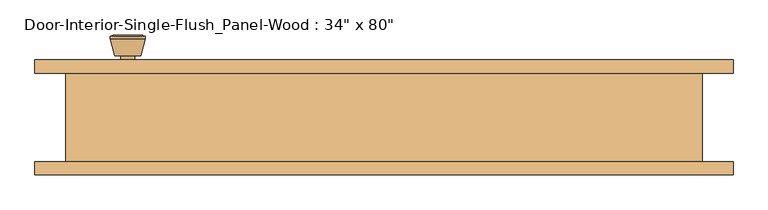
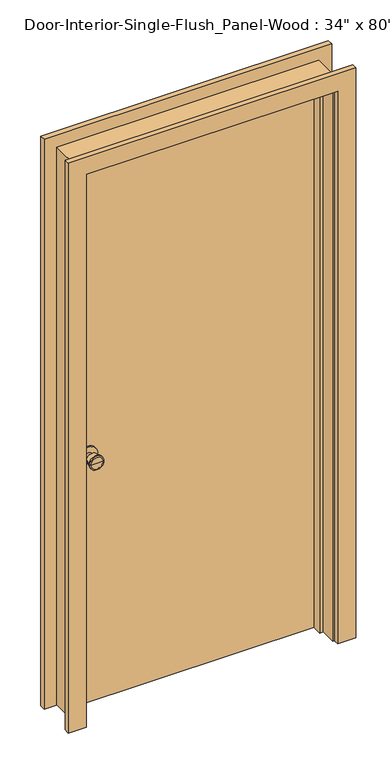
"""IFC4 building model written with IfcOpenShell, lengths in millimetres: door geometry."""

import ifcopenshell
import ifcopenshell.guid

model = None  # the IFC model being written
_history = None  # IfcOwnerHistory: only IFC2X3 demands one
_inside = {}  # id of a spatial element -> (the spatial element, [elements in it])
_under = {}  # id of a project, library or spatial element -> (it, [spatial elements below it])
_declared = {}  # id of a project -> (the project, [libraries it declares])
_typed = {}  # id of a type object -> (the type object, [elements of that type])
_made_of = {}  # id of a material, layer set ... -> (it, [elements and type objects made of it])


def new_model(schema):
    """Start an empty IFC model of exactly this schema.

    Asked for "IFC4X3", IfcOpenShell would pick the latest addendum, in which some entities
    have other attributes; the version numbers below select the first issue.
    IFC2X3 requires an IfcOwnerHistory on every rooted entity: one is made here for all.
    """
    global model, _history
    if schema == "IFC4X3":
        model = ifcopenshell.file(schema_version=(4, 3, 0, 0))
    else:
        model = ifcopenshell.file(schema=schema)
    _inside.clear()
    _under.clear()
    _declared.clear()
    _typed.clear()
    _made_of.clear()
    _history = None
    if model.schema == "IFC2X3":
        org = make("IfcOrganization", Name="unknown")
        user = make(
            "IfcPersonAndOrganization",
            ThePerson=make("IfcPerson", FamilyName="unknown"),
            TheOrganization=org,
        )
        app = make(
            "IfcApplication",
            ApplicationDeveloper=org,
            Version="unknown",
            ApplicationFullName="unknown",
            ApplicationIdentifier="unknown",
        )
        _history = make(
            "IfcOwnerHistory",
            OwningUser=user,
            OwningApplication=app,
            ChangeAction="ADDED",
            CreationDate=0,
        )
    return model


def make(cls, **values):
    """One entity of the class cls with the attributes given. An attribute that is None is left unset."""
    return model.create_entity(
        cls, **{name: value for name, value in values.items() if value is not None}
    )


def rooted(cls, **values):
    """An entity with a GlobalId (a new one), such as an element, a storey or a relation."""
    return make(cls, GlobalId=ifcopenshell.guid.new(), OwnerHistory=_history, **values)


def si_unit(unit_type, name, prefix=None):
    """IfcSIUnit, for example si_unit("LENGTHUNIT", "METRE", prefix="MILLI")."""
    return make("IfcSIUnit", UnitType=unit_type, Prefix=prefix, Name=name)


def assignment(units):
    """IfcUnitAssignment: the units of a project."""
    return None if units is None else make("IfcUnitAssignment", Units=units)


def point(xyz):
    """IfcCartesianPoint."""
    return None if xyz is None else make("IfcCartesianPoint", Coordinates=xyz)


def direction(xyz):
    """IfcDirection."""
    return None if xyz is None else make("IfcDirection", DirectionRatios=xyz)


def frame(location, z_axis=None, x_axis=None):
    """IfcAxis2Placement3D, a coordinate frame: its origin and axes. An axis left out is left unset."""
    return make(
        "IfcAxis2Placement3D",
        Location=point(location),
        Axis=direction(z_axis),
        RefDirection=direction(x_axis),
    )


def frame_2d(location, x_axis=None):
    """IfcAxis2Placement2D, a coordinate frame in the plane: its origin and x axis."""
    return make(
        "IfcAxis2Placement2D", Location=point(location), RefDirection=direction(x_axis)
    )


def origin():
    """The frame at (0, 0, 0) with its axes left unset."""
    return frame((0.0, 0.0, 0.0))


def origin_with_axes():
    """The frame at (0, 0, 0) with the z axis (0, 0, 1) and the x axis (1, 0, 0) written out."""
    return frame((0.0, 0.0, 0.0), z_axis=(0.0, 0.0, 1.0), x_axis=(1.0, 0.0, 0.0))


def place(relative_to, where):
    """IfcLocalPlacement: puts the frame where relative to a parent placement (None: the world)."""
    return make(
        "IfcLocalPlacement", PlacementRelTo=relative_to, RelativePlacement=where
    )


def context(
    kind, dimensions, precision=None, world=None, true_north=None, identifier=None
):
    """IfcGeometricRepresentationContext, for example the 3D "Model" context."""
    return make(
        "IfcGeometricRepresentationContext",
        ContextIdentifier=identifier,
        ContextType=kind,
        CoordinateSpaceDimension=dimensions,
        Precision=precision,
        WorldCoordinateSystem=world,
        TrueNorth=true_north,
    )


def project(units=None, contexts=None):
    """IfcProject with its units and contexts."""
    return rooted(
        "IfcProject",
        Name="project",
        RepresentationContexts=contexts,
        UnitsInContext=assignment(units),
    )


def spatial(cls, under=None, at=None, **own):
    """A site, building, storey or space (cls), placed at a placement, below another one or the project."""
    s = rooted(cls, ObjectPlacement=at, **own)
    if under is not None:
        _under.setdefault(under.id(), (under, []))[1].append(s)
    return s


def polyline(points):
    """IfcPolyline through the points."""
    return make("IfcPolyline", Points=[point(p) for p in points])


def circle_curve(where, radius):
    """IfcCircle in the frame where."""
    return make("IfcCircle", Position=where, Radius=radius)


def trimmed(basis, trim1, trim2, sense, master):
    """IfcTrimmedCurve: the piece of a basis curve between two trims."""
    return make(
        "IfcTrimmedCurve",
        BasisCurve=basis,
        Trim1=trim1,
        Trim2=trim2,
        SenseAgreement=sense,
        MasterRepresentation=master,
    )


def segment(curve, same_sense, transition):
    """IfcCompositeCurveSegment."""
    return make(
        "IfcCompositeCurveSegment",
        Transition=transition,
        SameSense=same_sense,
        ParentCurve=curve,
    )


def composite_curve(segments, self_intersect=None):
    """IfcCompositeCurve: segments joined end to end."""
    return make("IfcCompositeCurve", Segments=segments, SelfIntersect=self_intersect)


def outline(outer, holes=None, kind="AREA"):
    """IfcArbitraryClosedProfileDef: a profile drawn as a closed curve; with holes, ...WithVoids."""
    if holes is None:
        return make("IfcArbitraryClosedProfileDef", ProfileType=kind, OuterCurve=outer)
    return make(
        "IfcArbitraryProfileDefWithVoids",
        ProfileType=kind,
        OuterCurve=outer,
        InnerCurves=holes,
    )


def extrude(swept, where, along, depth):
    """IfcExtrudedAreaSolid: the profile swept, set in the frame where, extruded along a direction by depth."""
    return make(
        "IfcExtrudedAreaSolid",
        SweptArea=swept,
        Position=where,
        ExtrudedDirection=direction(along),
        Depth=depth,
    )


def faces_of(points, faces, orient=None, outer=None):
    """IfcFace entities. A face is a list of loops; a loop is a list of indices into points, from 0.

    orient and outer hold one flag for each loop. By default every Orientation is true, the
    first loop of a face is its IfcFaceOuterBound and the others are IfcFaceBound.
    """
    made = []
    for i, loops in enumerate(faces):
        bounds = []
        for j, loop in enumerate(loops):
            is_outer = j == 0 if outer is None else outer[i][j]
            bounds.append(
                make(
                    "IfcFaceOuterBound" if is_outer else "IfcFaceBound",
                    Bound=make("IfcPolyLoop", Polygon=[points[k] for k in loop]),
                    Orientation=True if orient is None else orient[i][j],
                )
            )
        made.append(make("IfcFace", Bounds=bounds))
    return made


def faceted_brep(points, faces, orient=None, outer=None, voids=None):
    """IfcFacetedBrep: a solid bounded by flat faces; with voids (closed shells), ...WithVoids."""
    shared = [point(p) for p in points]
    hull = make("IfcClosedShell", CfsFaces=faces_of(shared, faces, orient, outer))
    if voids is None:
        return make("IfcFacetedBrep", Outer=hull)
    return make(
        "IfcFacetedBrepWithVoids",
        Outer=hull,
        Voids=[
            make(cls, CfsFaces=faces_of(shared, fs, o, b)) for cls, fs, o, b in voids
        ],
    )


def shape(context_of_items, identifier, shape_type, items):
    """IfcShapeRepresentation: the items that make up one representation, for example the "Body"."""
    return make(
        "IfcShapeRepresentation",
        ContextOfItems=context_of_items,
        RepresentationIdentifier=identifier,
        RepresentationType=shape_type,
        Items=items,
    )


def source(mapping_origin, context_of_items, identifier, shape_type, items):
    """IfcRepresentationMap: a shape defined once, which mapped items show again and again."""
    return make(
        "IfcRepresentationMap",
        MappingOrigin=mapping_origin,
        MappedRepresentation=shape(context_of_items, identifier, shape_type, items),
    )


def transform(
    local_origin,
    x_axis=None,
    y_axis=None,
    z_axis=None,
    scale=None,
    scale2=None,
    scale3=None,
    uniform=True,
):
    """IfcCartesianTransformationOperator3D, or its non-uniform kind. x_axis, y_axis, z_axis: its Axis1, 2, 3."""
    if uniform:
        return make(
            "IfcCartesianTransformationOperator3D",
            Axis1=direction(x_axis),
            Axis2=direction(y_axis),
            LocalOrigin=point(local_origin),
            Scale=scale,
            Axis3=direction(z_axis),
        )
    return make(
        "IfcCartesianTransformationOperator3DnonUniform",
        Axis1=direction(x_axis),
        Axis2=direction(y_axis),
        LocalOrigin=point(local_origin),
        Scale=scale,
        Axis3=direction(z_axis),
        Scale2=scale2,
        Scale3=scale3,
    )


def mapped(mapping_source, mapping_target):
    """IfcMappedItem: shows the shape of a source again, moved by a transform."""
    return make(
        "IfcMappedItem", MappingSource=mapping_source, MappingTarget=mapping_target
    )


def made_of(thing, what):
    """Note that an element or type object is made of a material, layer set ...; save() writes the relation."""
    if what is not None:
        _made_of.setdefault(what.id(), (what, []))[1].append(thing)
    return thing


def element(
    cls,
    number,
    at=None,
    inside=None,
    cuts=None,
    type_object=None,
    material=None,
    context=None,
    identifier="Body",
    shape_type=None,
    held_by="IfcProductDefinitionShape",
    body=None,
    shapes=None,
    **own,
):
    """One element of the class cls, such as IfcWall. Its Tag is "e" and its number.

    at: its placement. inside: the storey or other place that contains it. cuts: it is an
    opening in that element (IfcRelVoidsElement). A single representation is given by context,
    identifier, shape_type and body (its items); several are given by shapes. held_by: the class
    of the entity that holds the representations. save() writes the other relations.
    """
    e = rooted(cls, Tag="e%d" % number, ObjectPlacement=at, **own)
    if body is not None:
        shapes = [shape(context, identifier, shape_type, body)]
    if shapes is not None:
        e.Representation = make(held_by, Representations=shapes)
    if inside is not None:
        _inside.setdefault(inside.id(), (inside, []))[1].append(e)
    if cuts is not None:
        rooted(
            "IfcRelVoidsElement", RelatingBuildingElement=cuts, RelatedOpeningElement=e
        )
    if type_object is not None:
        _typed.setdefault(type_object.id(), (type_object, []))[1].append(e)
    return made_of(e, material)


def aggregate(whole, parts):
    """IfcRelAggregates: a whole, such as a stair, and the parts it consists of."""
    return rooted("IfcRelAggregates", RelatingObject=whole, RelatedObjects=parts)


def save(model, path):
    """Write the relations noted so far, then the file.

    IfcRelAggregates (storeys below a building ...), IfcRelContainedInSpatialStructure (elements
    in a storey), IfcRelDefinesByType, IfcRelAssociatesMaterial and IfcRelDeclares: one each for
    every whole, place, type object, material and project.
    """
    for whole, parts in _under.values():
        aggregate(whole, parts)
    for where, things in _inside.values():
        rooted(
            "IfcRelContainedInSpatialStructure",
            RelatedElements=things,
            RelatingStructure=where,
        )
    for kind, things in _typed.values():
        rooted("IfcRelDefinesByType", RelatedObjects=things, RelatingType=kind)
    for what, things in _made_of.values():
        rooted("IfcRelAssociatesMaterial", RelatedObjects=things, RelatingMaterial=what)
    for by, libraries in _declared.values():
        rooted("IfcRelDeclares", RelatingContext=by, RelatedDefinitions=libraries)
    model.write(path)


def plane_surface(at):
    """IfcPlane: the flat surface through the origin of the frame at, square to its z axis."""
    return make("IfcPlane", Position=at)


def cylinder_surface(at, radius):
    """IfcCylindricalSurface: all points at the distance radius from the z axis of the frame at."""
    return make("IfcCylindricalSurface", Position=at, Radius=radius)


def revolved_surface(curve, axis_point, axis_direction):
    """IfcSurfaceOfRevolution: the curve turned about the line through axis_point along axis_direction."""
    return make(
        "IfcSurfaceOfRevolution",
        SweptCurve=make("IfcArbitraryOpenProfileDef", ProfileType="CURVE", Curve=curve),
        AxisPosition=make("IfcAxis1Placement", Location=point(axis_point), Axis=direction(axis_direction)),
    )


def advanced_brep(points, edges, surfaces, faces):
    """IfcAdvancedBrep: a solid bounded by faces that lie on surfaces and meet in shared edges.

    An edge is (start, end): straight between two places in points (the first is 0);
    or (start, end, curve); or (start, end, curve, False) where it runs against its curve.
    A face is (place in surfaces, loops), or (place, loops, False) where it looks against
    its surface's normal. A loop lists edges by number (the first is 1), with a minus sign
    where the edge is run from its end to its start. The first loop is the outer one.
    """
    corners = [point(p) for p in points]
    vertices = [make("IfcVertexPoint", VertexGeometry=c) for c in corners]
    made = []
    for start, end, *more in edges:
        made.append(
            make(
                "IfcEdgeCurve",
                EdgeStart=vertices[start],
                EdgeEnd=vertices[end],
                EdgeGeometry=more[0] if more else make("IfcPolyline", Points=[corners[start], corners[end]]),
                SameSense=more[1] if len(more) > 1 else True,
            )
        )
    hull = []
    for where, loops, *sense in faces:
        bounds = []
        for j, loop in enumerate(loops):
            ring = [make("IfcOrientedEdge", EdgeElement=made[abs(k) - 1], Orientation=k > 0) for k in loop]
            bounds.append(
                make(
                    "IfcFaceOuterBound" if j == 0 else "IfcFaceBound",
                    Bound=make("IfcEdgeLoop", EdgeList=ring),
                    Orientation=True,
                )
            )
        hull.append(make("IfcAdvancedFace", Bounds=bounds, FaceSurface=surfaces[where], SameSense=sense[0] if sense else True))
    return make("IfcAdvancedBrep", Outer=make("IfcClosedShell", CfsFaces=hull))


def door_5c12c2c5(model_context):
    return source(origin(), model_context, "Body", "SolidModel", [
        advanced_brep(
        [(-368.3, 19.4, 914.4), (-358.3, 19.4, 914.4), (-378.3, 19.4, 914.4), (-347.8241324, -29.6, 914.4), (-368.3, -29.6, 914.4), (-388.7758676, -29.6, 914.4), (-343.3, -27.7721319, 914.4), (-393.3, -27.7721319, 914.4), (-343.3, -24.3084537, 914.4), (-393.3, -24.3084537, 914.4), (-349.663764, 0.4, 914.4), (-386.936236, 0.4, 914.4), (-358.3, 0.4, 914.4), (-378.3, 0.4, 914.4)],
        [
            (0, 1),
            (1, 2, circle_curve(frame((-368.3, 19.4, 914.4), z_axis=(0.0, 1.0, 0.0), x_axis=(-1.0, 0.0, 0.0)), 10.0)),
            (2, 0),
            (2, 1, circle_curve(frame((-368.3, 19.4, 914.4), z_axis=(0.0, 1.0, 0.0), x_axis=(-1.0, 0.0, 0.0)), 10.0)),
            (3, 4),
            (4, 5),
            (5, 3, circle_curve(frame((-368.3, -29.6, 914.4), z_axis=(0.0, -1.0, 0.0), x_axis=(-1.0, 0.0, 0.0)), 20.4758676)),
            (3, 5, circle_curve(frame((-368.3, -29.6, 914.4), z_axis=(0.0, -1.0, 0.0), x_axis=(-1.0, 0.0, 0.0)), 20.4758676)),
            (6, 3),
            (5, 7),
            (7, 6, circle_curve(frame((-368.3, -27.7721319, 914.4), z_axis=(0.0, -1.0, 0.0), x_axis=(-1.0, 0.0, 0.0)), 25.0)),
            (6, 7, circle_curve(frame((-368.3, -27.7721319, 914.4), z_axis=(0.0, -1.0, 0.0), x_axis=(-1.0, 0.0, 0.0)), 25.0)),
            (8, 6),
            (7, 9),
            (9, 8, circle_curve(frame((-368.3, -24.3084537, 914.4), z_axis=(0.0, -1.0, 0.0), x_axis=(-1.0, 0.0, 0.0)), 25.0)),
            (8, 9, circle_curve(frame((-368.3, -24.3084537, 914.4), z_axis=(0.0, -1.0, 0.0), x_axis=(-1.0, 0.0, 0.0)), 25.0)),
            (10, 8),
            (9, 11),
            (11, 10, circle_curve(frame((-368.3, 0.4, 914.4), z_axis=(0.0, -1.0, 0.0), x_axis=(-1.0, 0.0, 0.0)), 18.636236)),
            (10, 11, circle_curve(frame((-368.3, 0.4, 914.4), z_axis=(0.0, -1.0, 0.0), x_axis=(-1.0, 0.0, 0.0)), 18.636236)),
            (12, 10),
            (11, 13),
            (13, 12, circle_curve(frame((-368.3, 0.4, 914.4), z_axis=(0.0, -1.0, 0.0), x_axis=(-1.0, 0.0, 0.0)), 10.0)),
            (12, 13, circle_curve(frame((-368.3, 0.4, 914.4), z_axis=(0.0, -1.0, 0.0), x_axis=(-1.0, 0.0, 0.0)), 10.0)),
            (1, 12),
            (13, 2),
        ],
        [
            plane_surface(frame((-368.3, 19.4, 914.4), z_axis=(0.0, 1.0, 0.0), x_axis=(-1.0, 0.0, 0.0))),
            plane_surface(frame((-368.3, -29.6, 914.4), z_axis=(0.0, -1.0, 0.0), x_axis=(-1.0, 0.0, 0.0))),
            revolved_surface(polyline([(-388.7758676, -29.6, 914.4), (-393.3, -27.7721319, 914.4)]), (-368.3, 19.4, 914.4), (0.0, 1.0, 0.0)),
            cylinder_surface(frame((-368.3, 19.4, 914.4), z_axis=(0.0, 1.0, 0.0), x_axis=(-1.0, 0.0, 0.0)), 25.0),
            revolved_surface(polyline([(-393.3, -24.3084537, 914.4), (-386.936236, 0.4, 914.4)]), (-368.3, 19.4, 914.4), (0.0, 1.0, 0.0)),
            plane_surface(frame((-368.3, 0.4, 914.4), z_axis=(0.0, 1.0, 0.0), x_axis=(-1.0, 0.0, 0.0))),
            cylinder_surface(frame((-368.3, 19.4, 914.4), z_axis=(0.0, 1.0, 0.0), x_axis=(-1.0, 0.0, 0.0)), 10.0),
        ],
        [
            (0, [[1, 2, 3]]),
            (0, [[-3, 4, -1]]),
            (1, [[5, 6, 7]]),
            (1, [[-6, -5, 8]]),
            (2, [[9, -7, 10, 11]]),
            (2, [[-10, -8, -9, 12]]),
            (3, [[13, -11, 14, 15]]),
            (3, [[-14, -12, -13, 16]]),
            (4, [[17, -15, 18, 19]]),
            (4, [[-18, -16, -17, 20]]),
            (5, [[21, -19, 22, 23]]),
            (5, [[-22, -20, -21, 24]]),
            (6, [[25, -23, 26, -2]]),
            (6, [[-26, -24, -25, -4]]),
        ],
    ),
        extrude(outline(composite_curve([segment(trimmed(circle_curve(frame_2d((914.4, -368.3)), 30.0), [point((914.4, -398.3))], [point((914.4, -338.3))], False, "CARTESIAN"), True, "CONTINUOUS"), segment(trimmed(circle_curve(frame_2d((914.4, -368.3)), 30.0), [point((914.4, -338.3))], [point((914.4, -398.3))], False, "CARTESIAN"), True, "CONTINUOUS")], self_intersect=False)), frame((0.0, 19.4, 0.0), z_axis=(0.0, 1.0, 0.0), x_axis=(0.0, 0.0, 1.0)), (0.0, 0.0, 1.0), 6.0),
        advanced_brep(
        [(-368.3, 66.325, 914.4), (-378.3, 66.325, 914.4), (-358.3, 66.325, 914.4), (-347.8241324, 115.325, 914.4), (-388.7758676, 115.325, 914.4), (-368.3, 115.325, 914.4), (-343.3, 113.4971319, 914.4), (-393.3, 113.4971319, 914.4), (-343.3, 110.0334537, 914.4), (-393.3, 110.0334537, 914.4), (-349.663764, 85.325, 914.4), (-386.936236, 85.325, 914.4), (-358.3, 85.325, 914.4), (-378.3, 85.325, 914.4)],
        [
            (0, 1),
            (1, 2, circle_curve(frame((-368.3, 66.325, 914.4), z_axis=(0.0, -1.0, 0.0), x_axis=(-1.0, 0.0, 0.0)), 10.0)),
            (2, 0),
            (2, 1, circle_curve(frame((-368.3, 66.325, 914.4), z_axis=(0.0, -1.0, 0.0), x_axis=(-1.0, 0.0, 0.0)), 10.0)),
            (3, 4, circle_curve(frame((-368.3, 115.325, 914.4), z_axis=(0.0, 1.0, 0.0), x_axis=(-1.0, 0.0, 0.0)), 20.4758676)),
            (4, 5),
            (5, 3),
            (4, 3, circle_curve(frame((-368.3, 115.325, 914.4), z_axis=(0.0, 1.0, 0.0), x_axis=(-1.0, 0.0, 0.0)), 20.4758676)),
            (6, 7, circle_curve(frame((-368.3, 113.4971319, 914.4), z_axis=(0.0, 1.0, 0.0), x_axis=(-1.0, 0.0, 0.0)), 25.0)),
            (7, 4),
            (3, 6),
            (7, 6, circle_curve(frame((-368.3, 113.4971319, 914.4), z_axis=(0.0, 1.0, 0.0), x_axis=(-1.0, 0.0, 0.0)), 25.0)),
            (8, 9, circle_curve(frame((-368.3, 110.0334537, 914.4), z_axis=(0.0, 1.0, 0.0), x_axis=(-1.0, 0.0, 0.0)), 25.0)),
            (9, 7),
            (6, 8),
            (9, 8, circle_curve(frame((-368.3, 110.0334537, 914.4), z_axis=(0.0, 1.0, 0.0), x_axis=(-1.0, 0.0, 0.0)), 25.0)),
            (10, 11, circle_curve(frame((-368.3, 85.325, 914.4), z_axis=(0.0, 1.0, 0.0), x_axis=(-1.0, 0.0, 0.0)), 18.636236)),
            (11, 9),
            (8, 10),
            (11, 10, circle_curve(frame((-368.3, 85.325, 914.4), z_axis=(0.0, 1.0, 0.0), x_axis=(-1.0, 0.0, 0.0)), 18.636236)),
            (12, 13, circle_curve(frame((-368.3, 85.325, 914.4), z_axis=(0.0, 1.0, 0.0), x_axis=(-1.0, 0.0, 0.0)), 10.0)),
            (13, 11),
            (10, 12),
            (13, 12, circle_curve(frame((-368.3, 85.325, 914.4), z_axis=(0.0, 1.0, 0.0), x_axis=(-1.0, 0.0, 0.0)), 10.0)),
            (1, 13),
            (12, 2),
        ],
        [
            plane_surface(frame((-368.3, 66.325, 914.4), z_axis=(0.0, -1.0, 0.0), x_axis=(-1.0, 0.0, 0.0))),
            plane_surface(frame((-368.3, 115.325, 914.4), z_axis=(0.0, 1.0, 0.0), x_axis=(-1.0, 0.0, 0.0))),
            revolved_surface(polyline([(-388.7758676, 115.325, 914.4), (-393.3, 113.4971319, 914.4)]), (-368.3, 66.325, 914.4), (0.0, -1.0, 0.0)),
            cylinder_surface(frame((-368.3, 66.325, 914.4), z_axis=(0.0, -1.0, 0.0), x_axis=(-1.0, 0.0, 0.0)), 25.0),
            revolved_surface(polyline([(-393.3, 110.0334537, 914.4), (-386.936236, 85.325, 914.4)]), (-368.3, 66.325, 914.4), (0.0, -1.0, 0.0)),
            plane_surface(frame((-368.3, 85.325, 914.4), z_axis=(0.0, -1.0, 0.0), x_axis=(-1.0, 0.0, 0.0))),
            cylinder_surface(frame((-368.3, 66.325, 914.4), z_axis=(0.0, -1.0, 0.0), x_axis=(-1.0, 0.0, 0.0)), 10.0),
        ],
        [
            (0, [[1, 2, 3]]),
            (0, [[-3, 4, -1]]),
            (1, [[5, 6, 7]]),
            (1, [[8, -7, -6]]),
            (2, [[9, 10, -5, 11]]),
            (2, [[12, -11, -8, -10]]),
            (3, [[13, 14, -9, 15]]),
            (3, [[16, -15, -12, -14]]),
            (4, [[17, 18, -13, 19]]),
            (4, [[20, -19, -16, -18]]),
            (5, [[21, 22, -17, 23]]),
            (5, [[24, -23, -20, -22]]),
            (6, [[-2, 25, -21, 26]]),
            (6, [[-4, -26, -24, -25]]),
        ],
    ),
        extrude(outline(composite_curve([segment(trimmed(circle_curve(frame_2d((914.4, -368.3)), 30.0), [point((914.4, -398.3))], [point((914.4, -338.3))], False, "CARTESIAN"), True, "CONTINUOUS"), segment(trimmed(circle_curve(frame_2d((914.4, -368.3)), 30.0), [point((914.4, -338.3))], [point((914.4, -398.3))], False, "CARTESIAN"), True, "CONTINUOUS")], self_intersect=False)), frame((0.0, 60.325, 0.0), z_axis=(0.0, 1.0, 0.0), x_axis=(0.0, 0.0, 1.0)), (0.0, 0.0, 1.0), 6.0),
        extrude(outline(polyline([(431.8, 25.4), (-431.8, 25.4), (-431.8, 60.325), (431.8, 60.325), (431.8, 25.4)])), origin_with_axes(), (0.0, 0.0, 1.0), 2032.0),
        faceted_brep([(457.2, 60.325, 0.0), (457.2, -66.675, 0.0), (431.8, -66.675, 0.0), (431.8, -9.525, 0.0), (419.1, -9.525, 0.0), (419.1, 25.4, 0.0), (431.8, 25.4, 0.0), (431.8, 60.325, 0.0), (457.2, 60.325, 2057.4), (457.2, -66.675, 2057.4), (-457.2, -66.675, 2057.4), (-457.2, -66.675, 0.0), (-431.8, -66.675, 0.0), (-431.8, -66.675, 2032.0), (431.8, -66.675, 2032.0), (431.8, -9.525, 2032.0), (-431.8, -9.525, 2032.0), (-431.8, -9.525, 0.0), (-419.1, -9.525, 0.0), (-419.1, -9.525, 2019.3), (419.1, -9.525, 2019.3), (419.1, 25.4, 2019.3), (-419.1, 25.4, 2019.3), (-419.1, 25.4, 0.0), (-431.8, 25.4, 0.0), (-431.8, 25.4, 2032.0), (431.8, 25.4, 2032.0), (431.8, 60.325, 2032.0), (-431.8, 60.325, 2032.0), (-431.8, 60.325, 0.0), (-457.2, 60.325, 0.0), (-457.2, 60.325, 2057.4)], [[[0, 1, 2, 3, 4, 5, 6, 7]], [[1, 0, 8, 9]], [[2, 1, 9, 10, 11, 12, 13, 14]], [[3, 2, 14, 15]], [[4, 3, 15, 16, 17, 18, 19, 20]], [[5, 4, 20, 21]], [[6, 5, 21, 22, 23, 24, 25, 26]], [[7, 6, 26, 27]], [[0, 7, 27, 28, 29, 30, 31, 8]], [[9, 8, 31, 10]], [[15, 14, 13, 16]], [[21, 20, 19, 22]], [[27, 26, 25, 28]], [[30, 29, 24, 23, 18, 17, 12, 11]], [[10, 31, 30, 11]], [[16, 13, 12, 17]], [[22, 19, 18, 23]], [[28, 25, 24, 29]]]),
        extrude(outline(polyline([(0.0, 438.15), (0.0, 501.65), (2101.85, 501.65), (2101.85, -501.65), (0.0, -501.65), (0.0, -438.15), (2038.35, -438.15), (2038.35, 438.15), (0.0, 438.15)])), frame((0.0, -85.725, 0.0), z_axis=(0.0, 1.0, 0.0), x_axis=(0.0, 0.0, 1.0)), (0.0, 0.0, 1.0), 19.05),
        extrude(outline(polyline([(0.0, 438.15), (0.0, 501.65), (2101.85, 501.65), (2101.85, -501.65), (0.0, -501.65), (0.0, -438.15), (2038.35, -438.15), (2038.35, 438.15), (0.0, 438.15)])), frame((0.0, 60.325, 0.0), z_axis=(0.0, 1.0, 0.0), x_axis=(0.0, 0.0, 1.0)), (0.0, 0.0, 1.0), 19.05),
    ])


if __name__ == "__main__":
    model = new_model("IFC4")
    model_context = context("Model", 3, world=origin())
    ifc_project = project(units=[si_unit("LENGTHUNIT", "METRE", prefix="MILLI")], contexts=[model_context])
    site = spatial("IfcSite", under=ifc_project)
    building = spatial("IfcBuilding", under=site)
    placement = place(None, origin())
    door_shape = door_5c12c2c5(model_context)
    element("IfcDoor", 1, ObjectType="Door-Interior-Single-Flush_Panel-Wood : 34\" x 80\"", at=placement, inside=building, context=model_context, shape_type="MappedRepresentation", body=[
        mapped(door_shape, transform((0.0, 0.0, 0.0), x_axis=(1.0, 0.0, 0.0), y_axis=(0.0, 1.0, 0.0), z_axis=(0.0, 0.0, 1.0))),
    ])
    save(model, "model.ifc")

# Revit data of these elements
# Type "Door-Interior-Single-Flush_Panel-Wood : 34\" x 80\""
#   Type Mark = "bb"
#   Assembly Code = "C1020300"
#   Analytic Construction = "Wooden"
#   Thickness = 0' - 1 3/8"
#   Thermal Resistance (R) = 0.455703 (m²·K)/W
#   Swing Angle [instance default] = 90.00°
#   Rough Width = 3' - 0"
#   Rough Height = 6' - 9"
#   Height = 6' - 8"
#   Width = 2' - 10"
#   Heat Transfer Coefficient (U) = 2.19465 W/(m²·K)
#   Trim Material = Cherry
#   Panel Material = Cherry
#   Frame Material = Cherry
#   Door Handle Material = Aluminum
#   Visual Light Transmittance = 0
#   Solar Heat Gain Coefficient = 0
#   Wall Closure = (empty or 0)
#   Function = (empty or 0)
# Element 1 (IfcDoor, "Door-Interior-Single-Flush_Panel-Wood : 34\" x 80\"")
#   Materials on its faces: "Cherry", "Aluminum"
# Materials
#   "Cherry": class "Wood", colour RGB 154 107 61, transparency 0, Description = "Prunus Serotina", Cost = 0
#   "Aluminum": class "Metal", colour RGB 244 244 244, transparency 0, Description = "Aluminum 6061", Cost = 0
